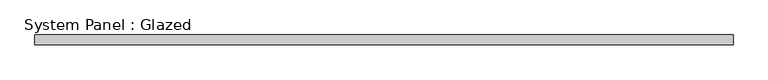
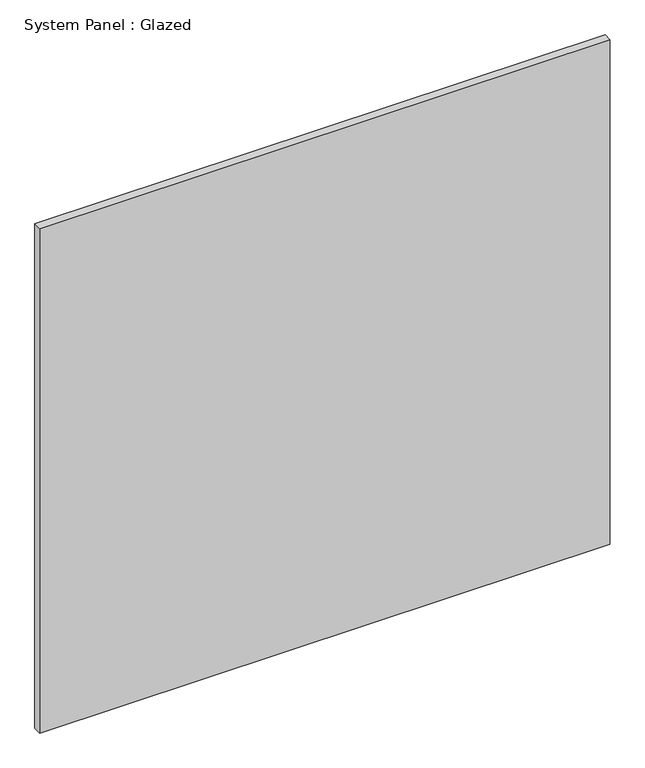
"""IFC4 building model written with IfcOpenShell, lengths in millimetres: plate geometry, System Panel : Glazed."""

from ifc_helpers import new_model, si_unit, origin, origin_with_axes, place, context, project, spatial, polyline, outline, extrude, source, transform, mapped, element, save


def system_panel_glazed_95db9f90(model_context):
    return source(origin(), model_context, "Body", "SweptSolid", [
        extrude(outline(polyline([(877.5000002, 24.5), (-877.5000002, 24.5), (-877.5000002, 49.5), (877.5000002, 49.5), (877.5000002, 24.5)])), origin_with_axes(), (0.0, 0.0, 1.0), 1640.2939092),
    ])


if __name__ == "__main__":
    model = new_model("IFC4")
    model_context = context("Model", 3, world=origin())
    ifc_project = project(units=[si_unit("LENGTHUNIT", "METRE", prefix="MILLI")], contexts=[model_context])
    site = spatial("IfcSite", under=ifc_project)
    building = spatial("IfcBuilding", under=site)
    placement = place(None, origin())
    system_panel_glazed_shape = system_panel_glazed_95db9f90(model_context)
    element("IfcPlate", 1, ObjectType="System Panel : Glazed", at=placement, inside=building, context=model_context, shape_type="MappedRepresentation", body=[
        mapped(system_panel_glazed_shape, transform((0.0, 0.0, 0.0), x_axis=(1.0, 0.0, 0.0), y_axis=(0.0, 1.0, 0.0), z_axis=(0.0, 0.0, 1.0))),
    ])
    save(model, "model.ifc")

# Revit data of these elements
# Element 1 (IfcPlate, "System Panel : Glazed")
#   Materials on its faces: "Glass"
# Materials
#   "Glass": class "Glass", colour RGB 218 227 224, transparency 0.85, Description = "Soda Lime Glass", Cost = 0
